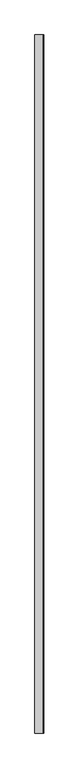
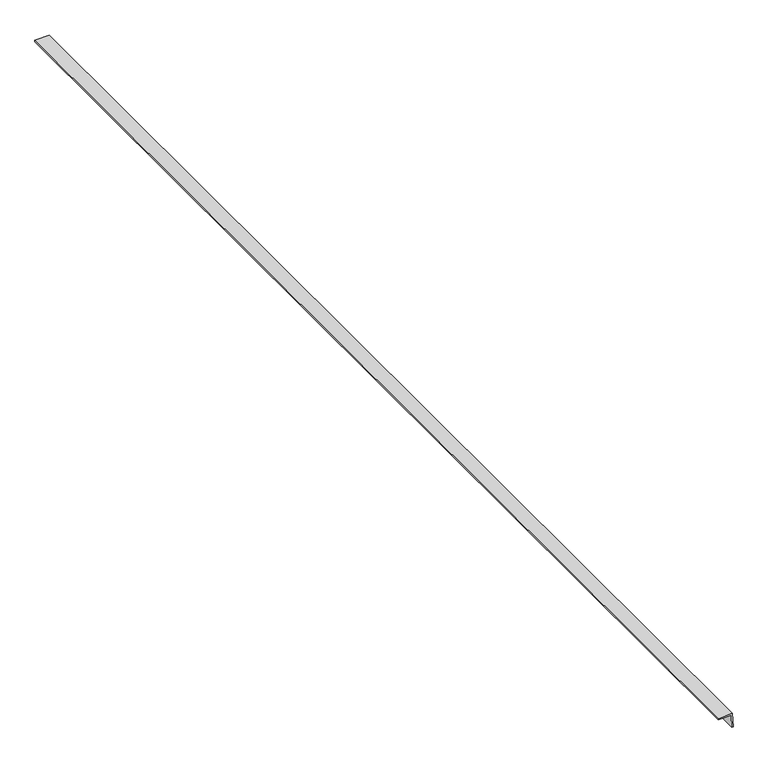
"""IFC4 building model written with IfcOpenShell, lengths in millimetres: proxy geometry, Generic Models 7:Generic Models 1:337419:Generic Models 1:337419 : Generic Models 7:Generic Models 1:337419:46 : Generic Models 7:Generic Models 1:337419:Generic Models 1:337419 : Generic Models 7:Generic Models 1:337419:301336."""

from ifc_helpers import new_model, si_unit, frame, origin, place, context, project, spatial, polyline, outline, extrude, source, transform, mapped, element, save


def generic_models_648b2253(model_context):
    return source(origin(), model_context, "Body", "SweptSolid", [
        extrude(outline(polyline([(4449.9168223, 579077.5233339), (4447.8019906, 579026.7673738), (4443.0436194, 579026.9656393), (4444.9601856, 579072.9632281), (4398.9625967, 579074.8797943), (4399.1608622, 579079.6381656), (4449.9168223, 579077.5233339)])), frame((0.0, -578797.4913841, 0.0), z_axis=(0.0, 1.0, 0.0), x_axis=(0.0, 0.0, 1.0)), (0.0, 0.0, 1.0), 4145.5624605),
    ])


if __name__ == "__main__":
    model = new_model("IFC4")
    model_context = context("Model", 3, world=origin())
    ifc_project = project(units=[si_unit("LENGTHUNIT", "METRE", prefix="MILLI")], contexts=[model_context])
    site = spatial("IfcSite", under=ifc_project)
    building = spatial("IfcBuilding", under=site)
    placement = place(None, origin())
    generic_models_shape = generic_models_648b2253(model_context)
    element("IfcBuildingElementProxy", 1, Name="Generic Models 7:Generic Models 1:337419:Generic Models 1:337419 : Generic Models 7:Generic Models 1:337419:46 : Generic Models 7:Generic Models 1:337419:Generic Models 1:337419 : Generic Models 7:Generic Models 1:337419:301336", ObjectType="Generic Models 7:Generic Models 1:337419:Generic Models 1:337419 : Generic Models 7:Generic Models 1:337419:46 : Generic Models 7:Generic Models 1:337419:Generic Models 1:337419 : Generic Models 7:Generic Models 1:337419:301336", at=placement, inside=building, context=model_context, shape_type="MappedRepresentation", body=[
        mapped(generic_models_shape, transform((0.0, 0.0, 0.0), x_axis=(1.0, 0.0, 0.0), y_axis=(0.0, 1.0, 0.0), z_axis=(0.0, 0.0, 1.0))),
    ])
    save(model, "model.ifc")

# Revit data of these elements
# Type "Generic Models 7:Generic Models 1:337419:Generic Models 1:337419 : Generic Models 7:Generic Models 1:337419:46 : Generic Models 7:Generic Models 1:337419:Generic Models 1:337419 : Generic Models 7:Generic Models 1:337419:301336"
#   NameOverride = "Generic Models 7:Generic Models 1:337419:Generic Models 1:337419 : Generic Models 7:Generic Models 1:337419:301336"
#   ObjectTypeOverride = "Generic Models 1:337419 : Generic Models 7:Generic Models 1:337419"
#   Reference = "Generic Models 1"
#   Tag = "301336"
# Element 1 (IfcBuildingElementProxy, "Generic Models 7:Generic Models 1:337419:Generic Models 1:337419 : Generic Models 7:Generic Models 1:337419:46 : Generic Models 7:Generic Models 1:337419:Generic Models 1:337419 : Generic Models 7:Generic Models 1:337419:301336")
#   Materials on its faces: "2 X 2 X 3/16 GAL. STEEL ANGLE TO FASTEN INTERIOR PLYWOOD."
# Materials
#   "2 X 2 X 3/16 GAL. STEEL ANGLE TO FASTEN INTERIOR PLYWOOD.": class "Unassigned", colour RGB 210 209 208, transparency 0, Keynote = "M05121300.02", Cost = 0
